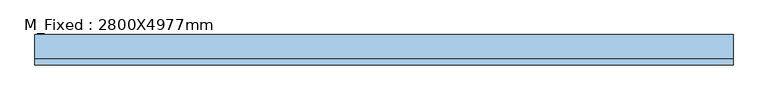
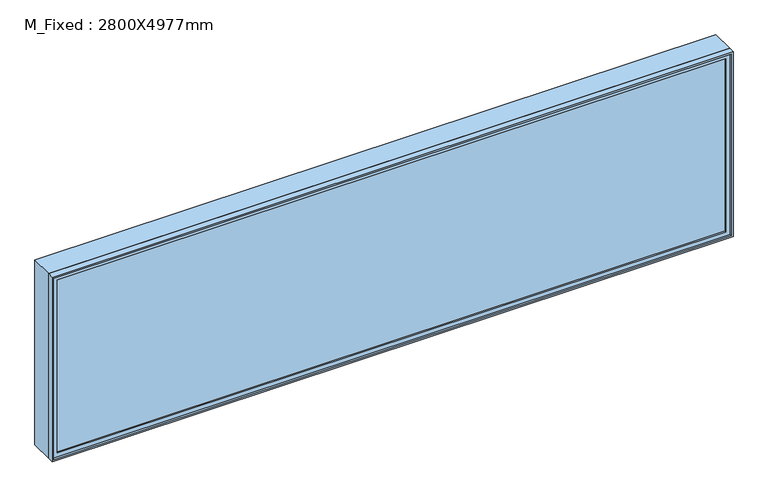
"""IFC4 building model written with IfcOpenShell, lengths in millimetres: window geometry, M_Fixed : 2800X4977mm."""

from ifc_helpers import new_model, si_unit, frame, origin, place, context, project, spatial, polyline, outline, extrude, source, transform, mapped, element, save


def m_fixed_2800x4977mm_bf86b0e8(model_context):
    return source(origin(), model_context, "Body", "SweptSolid", [
        extrude(outline(polyline([(-3420.85, -130.4), (-3420.85, -118.4), (3420.85, -118.4), (3420.85, -130.4), (-3420.85, -130.4)])), frame((0.0, 0.0, 978.0), z_axis=(0.0, 0.0, 1.0), x_axis=(1.0, 0.0, 0.0)), (0.0, 0.0, 1.0), 1874.0),
        extrude(outline(polyline([(2896.0, -3464.85), (934.0, -3464.85), (934.0, 3464.85), (2896.0, 3464.85), (2896.0, -3464.85)]), holes=[polyline([(2852.0, -3420.85), (2852.0, 3420.85), (978.0, 3420.85), (978.0, -3420.85), (2852.0, -3420.85)])]), frame((0.0, -146.4, 0.0), z_axis=(0.0, 1.0, 0.0), x_axis=(0.0, 0.0, 1.0)), (0.0, 0.0, 1.0), 44.0),
        extrude(outline(polyline([(2915.0, -3483.85), (915.0, -3483.85), (915.0, 3483.85), (2915.0, 3483.85), (2915.0, -3483.85)]), holes=[polyline([(2896.0, -3464.85), (2896.0, 3464.85), (934.0, 3464.85), (934.0, -3464.85), (2896.0, -3464.85)])]), frame((0.0, -165.4, 0.0), z_axis=(0.0, 1.0, 0.0), x_axis=(0.0, 0.0, 1.0)), (0.0, 0.0, 1.0), 63.0),
        extrude(outline(polyline([(2915.0, -3483.85), (915.0, -3483.85), (915.0, 3483.85), (2915.0, 3483.85), (2915.0, -3483.85)]), holes=[polyline([(2883.0, -3451.85), (2883.0, 3451.85), (947.0, 3451.85), (947.0, -3451.85), (2883.0, -3451.85)])]), frame((0.0, -102.4, 0.0), z_axis=(0.0, 1.0, 0.0), x_axis=(0.0, 0.0, 1.0)), (0.0, 0.0, 1.0), 241.8),
    ])


if __name__ == "__main__":
    model = new_model("IFC4")
    model_context = context("Model", 3, world=origin())
    ifc_project = project(units=[si_unit("LENGTHUNIT", "METRE", prefix="MILLI")], contexts=[model_context])
    site = spatial("IfcSite", under=ifc_project)
    building = spatial("IfcBuilding", under=site)
    placement = place(None, origin())
    m_fixed_2800x4977mm_shape = m_fixed_2800x4977mm_bf86b0e8(model_context)
    element("IfcWindow", 1, ObjectType="M_Fixed : 2800X4977mm", at=placement, inside=building, context=model_context, shape_type="MappedRepresentation", body=[
        mapped(m_fixed_2800x4977mm_shape, transform((0.0, 0.0, 0.0), x_axis=(1.0, 0.0, 0.0), y_axis=(0.0, 1.0, 0.0), z_axis=(0.0, 0.0, 1.0))),
    ])
    save(model, "model.ifc")

# Revit data of these elements
# Type "M_Fixed : 2800X4977mm"
#   Type Mark = "29"
#   Height = 2000 mm
#   Default Sill Height = 915 mm
#   Width = 6967.7 mm
#   Window Inset = 19 mm
#   Frame Exterior Material = Sash
#   Frame Interior Material = Sash
#   Glass Pane Material = Glass
#   Sash = Sash
#   Wall Closure = (empty or 0)
# Element 1 (IfcWindow, "M_Fixed : 2800X4977mm")
#   Materials on its faces: "Sash", "Glass"
# Materials
#   "Sash": class "Wood", colour RGB 136 99 55, transparency 0
#   "Glass": class "Glass", colour RGB 0 128 192, transparency 0.9, Description = "Soda Lime Glass", Cost = 0
